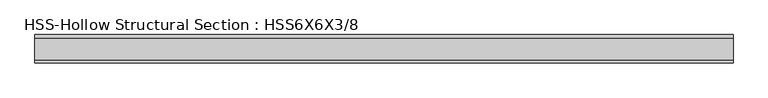
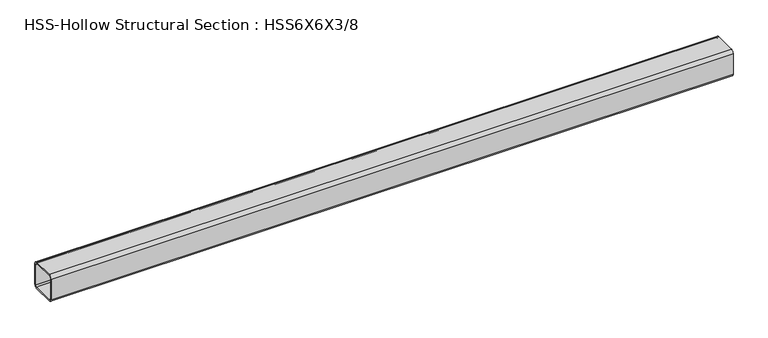
"""IFC4 building model written with IfcOpenShell, lengths in millimetres: member geometry, HSS-Hollow Structural Section : HSS6X6X3/8."""

from ifc_helpers import new_model, si_unit, point, frame, frame_2d, origin, place, context, project, spatial, polyline, circle_curve, trimmed, segment, composite_curve, outline, extrude, source, transform, mapped, element, save


def hss_hollow_structural_section_hss6x6x3_8_68fbf6d9(model_context):
    return source(origin(), model_context, "Body", "SweptSolid", [
        extrude(outline(composite_curve([segment(polyline([(76.2, 58.4708), (76.2, -58.4708)]), True, "CONTINUOUS"), segment(trimmed(circle_curve(frame_2d((58.4708, -58.4708)), 17.7292), [point((76.2, -58.4708))], [point((58.4708, -76.2))], False, "CARTESIAN"), True, "CONTINUOUS"), segment(polyline([(58.4708, -76.2), (-58.4708, -76.2)]), True, "CONTINUOUS"), segment(trimmed(circle_curve(frame_2d((-58.4708, -58.4708)), 17.7292), [point((-58.4708, -76.2))], [point((-76.2, -58.4708))], False, "CARTESIAN"), True, "CONTINUOUS"), segment(polyline([(-76.2, -58.4708), (-76.2, 58.4708)]), True, "CONTINUOUS"), segment(trimmed(circle_curve(frame_2d((-58.4708, 58.4708)), 17.7292), [point((-76.2, 58.4708))], [point((-58.4708, 76.2))], False, "CARTESIAN"), True, "CONTINUOUS"), segment(polyline([(-58.4708, 76.2), (58.4708, 76.2)]), True, "CONTINUOUS"), segment(trimmed(circle_curve(frame_2d((58.4708, 58.4708)), 17.7292), [point((58.4708, 76.2))], [point((76.2, 58.4708))], False, "CARTESIAN"), True, "CONTINUOUS")], self_intersect=False), holes=[composite_curve([segment(trimmed(circle_curve(frame_2d((-58.4708, 58.4708)), 8.8646), [point((-58.4708, 67.3354))], [point((-67.3354, 58.4708))], True, "CARTESIAN"), True, "CONTINUOUS"), segment(polyline([(-67.3354, 58.4708), (-67.3354, -58.4708)]), True, "CONTINUOUS"), segment(trimmed(circle_curve(frame_2d((-58.4708, -58.4708)), 8.8646), [point((-67.3354, -58.4708))], [point((-58.4708, -67.3354))], True, "CARTESIAN"), True, "CONTINUOUS"), segment(polyline([(-58.4708, -67.3354), (58.4708, -67.3354)]), True, "CONTINUOUS"), segment(trimmed(circle_curve(frame_2d((58.4708, -58.4708)), 8.8646), [point((58.4708, -67.3354))], [point((67.3354, -58.4708))], True, "CARTESIAN"), True, "CONTINUOUS"), segment(polyline([(67.3354, -58.4708), (67.3354, 58.4708)]), True, "CONTINUOUS"), segment(trimmed(circle_curve(frame_2d((58.4708, 58.4708)), 8.8646), [point((67.3354, 58.4708))], [point((58.4708, 67.3354))], True, "CARTESIAN"), True, "CONTINUOUS"), segment(polyline([(58.4708, 67.3354), (-58.4708, 67.3354)]), True, "CONTINUOUS")], self_intersect=False)]), frame((-1760.5837481, 0.0, 0.0), z_axis=(1.0, 0.0, 0.0), x_axis=(0.0, 1.0, 0.0)), (0.0, 0.0, 1.0), 3725.9173358),
    ])


if __name__ == "__main__":
    model = new_model("IFC4")
    model_context = context("Model", 3, world=origin())
    ifc_project = project(units=[si_unit("LENGTHUNIT", "METRE", prefix="MILLI")], contexts=[model_context])
    site = spatial("IfcSite", under=ifc_project)
    building = spatial("IfcBuilding", under=site)
    placement = place(None, origin())
    hss_hollow_structural_section_hss6x6x3_8_shape = hss_hollow_structural_section_hss6x6x3_8_68fbf6d9(model_context)
    element("IfcMember", 1, ObjectType="HSS-Hollow Structural Section : HSS6X6X3/8", at=placement, inside=building, context=model_context, shape_type="MappedRepresentation", body=[
        mapped(hss_hollow_structural_section_hss6x6x3_8_shape, transform((0.0, 0.0, 0.0), x_axis=(1.0, 0.0, 0.0), y_axis=(0.0, 1.0, 0.0), z_axis=(0.0, 0.0, 1.0))),
    ])
    save(model, "model.ifc")

# Revit data of these elements
# Type "HSS-Hollow Structural Section : HSS6X6X3/8"
#   Assembly Code = "B10"
#   Shape = "Square"
#   W = 27.4
#   Ht = 0' - 6"
#   Length [instance default] = 5' - 0"
#   b = 0' - 6"
#   kr = 0' - 0.698"
#   t = 0' - 0.349"
#   A = 0.0526389 SF
#   Structural Material [instance default] = Steel ASTM A500, Grade B, Rectangular and Square
# Element 1 (IfcMember, "HSS-Hollow Structural Section : HSS6X6X3/8")
#   Materials on its faces: "Steel ASTM A500, Grade B, Rectangular and Square"
# Materials
#   "Steel ASTM A500, Grade B, Rectangular and Square": class "Metal", colour RGB 199 199 199, transparency 0, Description = "Carbon steel", Cost = 0
